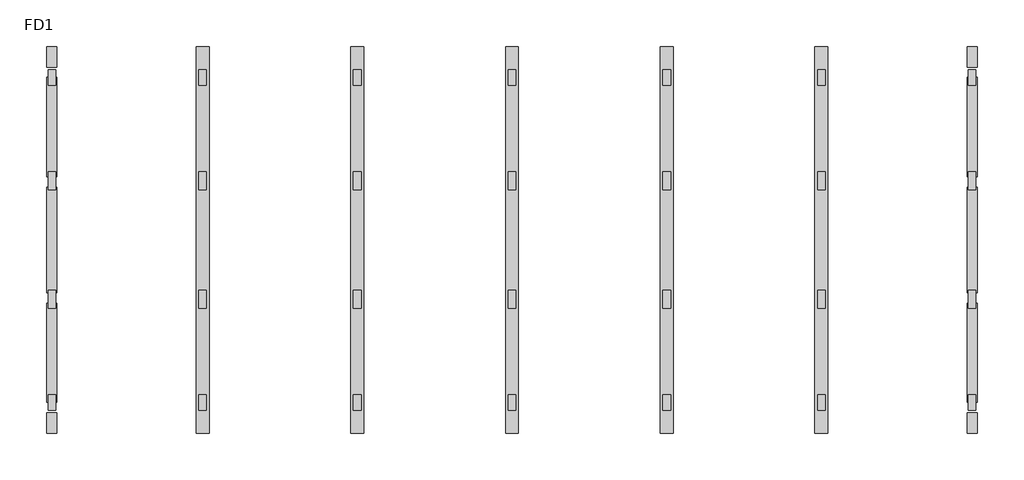
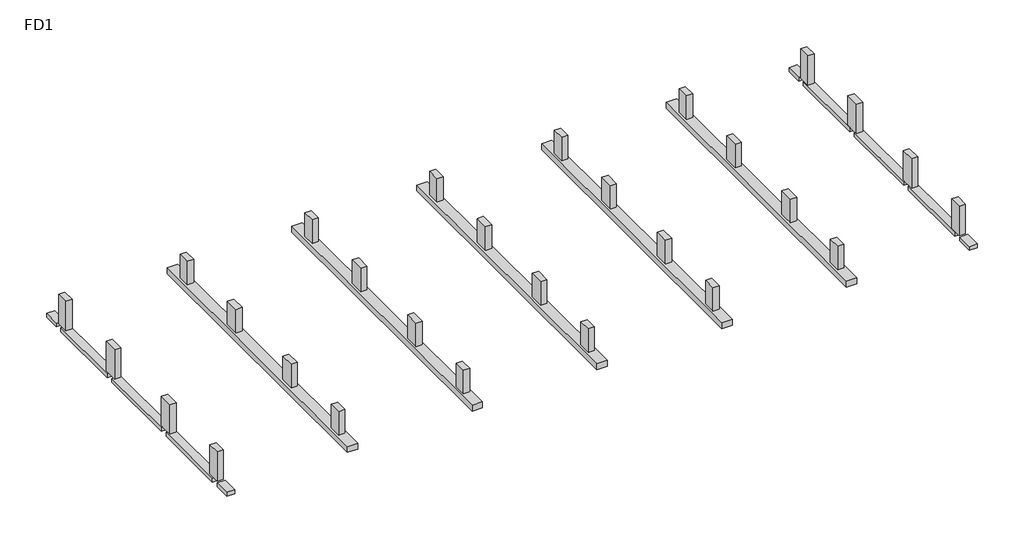
# One storey: 28 columns, 7 beams.
"""IFC4 building model written with IfcOpenShell, lengths in millimetres."""

from ifc_helpers import new_model, si_unit, frame, origin, place, context, project, spatial, polyline, outline, extrude, faceted_brep, element, save

model = new_model("IFC4")

# Units and contexts
model_context = context("Model", 3, world=origin())
ifc_project = project(units=[si_unit("LENGTHUNIT", "METRE", prefix="MILLI")], contexts=[model_context])

# Site, building, storey
site = spatial("IfcSite", under=ifc_project)
building = spatial("IfcBuilding", under=site)
storey = spatial("IfcBuildingStorey", under=building, Name="FD1", Elevation=-1170.0)

# Beams
placement = place(None, origin())
element("IfcBeam", 1, ObjectType="M_Concrete-Rectangular Beam : 400x700", at=placement, inside=storey, context=model_context, shape_type="SweptSolid", body=[
    extrude(outline(polyline([(35899.948043, -1000.0), (35499.948043, -1000.0), (35499.948043, -200.0), (35899.948043, -200.0), (35899.948043, -1000.0)])), frame((0.0, 0.0, -1670.0), z_axis=(0.0, 0.0, 1.0), x_axis=(1.0, 0.0, 0.0)), (0.0, 0.0, 1.0), 200.0),
    extrude(outline(polyline([(35499.948043, 14000.0000002), (35899.948043, 14000.0000002), (35899.948043, 13200.0000002), (35499.948043, 13200.0000002), (35499.948043, 14000.0000002)])), frame((0.0, 0.0, -1670.0), z_axis=(0.0, 0.0, 1.0), x_axis=(1.0, 0.0, 0.0)), (0.0, 0.0, 1.0), 200.0),
    extrude(outline(polyline([(35499.948043, 12800.0000002), (35899.948043, 12800.0000002), (35899.948043, 8950.0000002), (35499.948043, 8950.0000002), (35499.948043, 12800.0000002)])), frame((0.0, 0.0, -1670.0), z_axis=(0.0, 0.0, 1.0), x_axis=(1.0, 0.0, 0.0)), (0.0, 0.0, 1.0), 200.0),
    extrude(outline(polyline([(35499.948043, 8550.0000002), (35899.948043, 8550.0000002), (35899.948043, 4450.0000002), (35499.948043, 4450.0000002), (35499.948043, 8550.0000002)])), frame((0.0, 0.0, -1670.0), z_axis=(0.0, 0.0, 1.0), x_axis=(1.0, 0.0, 0.0)), (0.0, 0.0, 1.0), 200.0),
    extrude(outline(polyline([(35499.948043, 4050.0000002), (35899.948043, 4050.0000002), (35899.948043, 200.0), (35499.948043, 200.0), (35499.948043, 4050.0000002)])), frame((0.0, 0.0, -1670.0), z_axis=(0.0, 0.0, 1.0), x_axis=(1.0, 0.0, 0.0)), (0.0, 0.0, 1.0), 200.0),
])
element("IfcBeam", 2, ObjectType="M_Concrete-Rectangular Beam : 400x700", at=placement, inside=storey, context=model_context, shape_type="SweptSolid", body=[
    extrude(outline(polyline([(200.0, -1000.0), (-200.0, -1000.0), (-200.0, -200.0), (200.0, -200.0), (200.0, -1000.0)])), frame((0.0, 0.0, -1670.0), z_axis=(0.0, 0.0, 1.0), x_axis=(1.0, 0.0, 0.0)), (0.0, 0.0, 1.0), 200.0),
    extrude(outline(polyline([(-200.0, 14000.0000002), (200.0, 14000.0000002), (200.0, 13200.0000002), (-200.0, 13200.0000002), (-200.0, 14000.0000002)])), frame((0.0, 0.0, -1670.0), z_axis=(0.0, 0.0, 1.0), x_axis=(1.0, 0.0, 0.0)), (0.0, 0.0, 1.0), 200.0),
    extrude(outline(polyline([(-200.0, 12800.0000002), (200.0, 12800.0000002), (200.0, 8950.0000002), (-200.0, 8950.0000002), (-200.0, 12800.0000002)])), frame((0.0, 0.0, -1670.0), z_axis=(0.0, 0.0, 1.0), x_axis=(1.0, 0.0, 0.0)), (0.0, 0.0, 1.0), 200.0),
    extrude(outline(polyline([(-200.0, 8550.0000002), (200.0, 8550.0000002), (200.0, 4450.0000002), (-200.0, 4450.0000002), (-200.0, 8550.0000002)])), frame((0.0, 0.0, -1670.0), z_axis=(0.0, 0.0, 1.0), x_axis=(1.0, 0.0, 0.0)), (0.0, 0.0, 1.0), 200.0),
    extrude(outline(polyline([(-200.0, 4050.0000002), (200.0, 4050.0000002), (200.0, 200.0), (-200.0, 200.0), (-200.0, 4050.0000002)])), frame((0.0, 0.0, -1670.0), z_axis=(0.0, 0.0, 1.0), x_axis=(1.0, 0.0, 0.0)), (0.0, 0.0, 1.0), 200.0),
])
element("IfcBeam", 3, ObjectType="M_Concrete-Rectangular Beam : 500x1000", at=placement, inside=storey, context=model_context, shape_type="SweptSolid", body=[
    extrude(outline(polyline([(29600.0000039, 14000.0000002), (30100.0000039, 14000.0000002), (30100.0000039, -1000.0), (29600.0000039, -1000.0), (29600.0000039, 14000.0000002)])), frame((0.0, 0.0, -1470.0), z_axis=(0.0, 0.0, 1.0), x_axis=(1.0, 0.0, 0.0)), (0.0, 0.0, 1.0), 300.0),
])
element("IfcBeam", 4, ObjectType="M_Concrete-Rectangular Beam : 500x1000", at=placement, inside=storey, context=model_context, shape_type="SweptSolid", body=[
    extrude(outline(polyline([(6100.0000012, -1000.0), (5600.0000012, -1000.0), (5600.0000012, 14000.0000002), (6100.0000012, 14000.0000002), (6100.0000012, -1000.0)])), frame((0.0, 0.0, -1470.0), z_axis=(0.0, 0.0, 1.0), x_axis=(1.0, 0.0, 0.0)), (0.0, 0.0, 1.0), 300.0),
])
element("IfcBeam", 5, ObjectType="M_Concrete-Rectangular Beam : 500x1000", at=placement, inside=storey, context=model_context, shape_type="Brep", body=[
    faceted_brep([(24100.0000056, -1000.0, -1170.0), (23600.0000056, -1000.0, -1170.0), (23600.0000056, -1000.0, -1469.9652093), (24100.0000056, -1000.0, -1470.0), (23600.0000056, 14000.0000002, -1170.0), (24100.0000056, 14000.0000002, -1170.0), (24100.0000056, 14000.0000002, -1470.0347907), (23600.0000056, 14000.0000002, -1470.0)], [[[0, 1, 2, 3]], [[4, 5, 6, 7]], [[1, 0, 5, 4]], [[1, 4, 7, 2]], [[5, 0, 3, 6]], [[3, 2, 7, 6]]]),
])
element("IfcBeam", 6, ObjectType="M_Concrete-Rectangular Beam : 500x1000", at=placement, inside=storey, context=model_context, shape_type="Brep", body=[
    faceted_brep([(18099.8537458, -1000.0, -1170.0), (17599.8537458, -1000.0, -1170.0), (17599.8537458, -1000.0, -1469.962184), (18099.8537458, -1000.0, -1470.0), (17599.8537458, 14000.0000002, -1170.0), (18099.8537458, 14000.0000002, -1170.0), (18099.8537458, 14000.0000002, -1470.037816), (17599.8537458, 14000.0000002, -1470.0)], [[[0, 1, 2, 3]], [[4, 5, 6, 7]], [[1, 0, 5, 4]], [[1, 4, 7, 2]], [[5, 0, 3, 6]], [[3, 2, 7, 6]]]),
])
element("IfcBeam", 7, ObjectType="M_Concrete-Rectangular Beam : 500x1000", at=placement, inside=storey, context=model_context, shape_type="Brep", body=[
    faceted_brep([(12100.0000006, -1000.0, -1170.0), (11600.0000006, -1000.0, -1170.0), (11600.0000006, -1000.0, -1469.9652093), (12100.0000006, -1000.0, -1470.0), (11600.0000006, 14000.0000002, -1170.0), (12100.0000006, 14000.0000002, -1170.0), (12100.0000006, 14000.0000002, -1470.0347907), (11600.0000006, 14000.0000002, -1470.0)], [[[0, 1, 2, 3]], [[4, 5, 6, 7]], [[1, 0, 5, 4]], [[1, 4, 7, 2]], [[5, 0, 3, 6]], [[3, 2, 7, 6]]]),
])

# Columns
element("IfcColumn", 8, ObjectType="M_Concrete-Rectangular-Column : 300x600", at=placement, inside=storey, context=model_context, shape_type="SweptSolid", body=[
    extrude(outline(polyline([(165.0, 499.9999998), (165.0, -100.0000002), (-135.0, -100.0000002), (-135.0, 499.9999998), (165.0, 499.9999998)])), frame((0.0, 0.0, -1470.0), z_axis=(0.0, 0.0, 1.0), x_axis=(1.0, 0.0, 0.0)), (0.0, 0.0, 1.0), 1500.0),
])
element("IfcColumn", 9, ObjectType="M_Concrete-Rectangular-Column : 300x600", at=placement, inside=storey, context=model_context, shape_type="SweptSolid", body=[
    extrude(outline(polyline([(164.9999993, 13100.0000003), (164.9999993, 12500.0000003), (-135.0000007, 12500.0000003), (-135.0000007, 13100.0000003), (164.9999993, 13100.0000003)])), frame((0.0, 0.0, -1470.0), z_axis=(0.0, 0.0, 1.0), x_axis=(1.0, 0.0, 0.0)), (0.0, 0.0, 1.0), 1500.0),
])
element("IfcColumn", 10, ObjectType="M_Concrete-Rectangular-Column : 300x600", at=placement, inside=storey, context=model_context, shape_type="SweptSolid", body=[
    extrude(outline(polyline([(6000.0000007, 499.9999998), (6000.0000007, -100.0000002), (5700.0000007, -100.0000002), (5700.0000007, 499.9999998), (6000.0000007, 499.9999998)])), frame((0.0, 0.0, -1170.0), z_axis=(0.0, 0.0, 1.0), x_axis=(1.0, 0.0, 0.0)), (0.0, 0.0, 1.0), 1200.0),
])
element("IfcColumn", 11, ObjectType="M_Concrete-Rectangular-Column : 300x600", at=placement, inside=storey, context=model_context, shape_type="SweptSolid", body=[
    extrude(outline(polyline([(12000.0000034, 499.9999998), (12000.0000034, -100.0000002), (11700.0000034, -100.0000002), (11700.0000034, 499.9999998), (12000.0000034, 499.9999998)])), frame((0.0, 0.0, -1170.0), z_axis=(0.0, 0.0, 1.0), x_axis=(1.0, 0.0, 0.0)), (0.0, 0.0, 1.0), 1200.0),
])
element("IfcColumn", 12, ObjectType="M_Concrete-Rectangular-Column : 300x600", at=placement, inside=storey, context=model_context, shape_type="SweptSolid", body=[
    extrude(outline(polyline([(18000.0000058, 499.9999998), (18000.0000058, -100.0000002), (17700.0000058, -100.0000002), (17700.0000058, 499.9999998), (18000.0000058, 499.9999998)])), frame((0.0, 0.0, -1170.0), z_axis=(0.0, 0.0, 1.0), x_axis=(1.0, 0.0, 0.0)), (0.0, 0.0, 1.0), 1200.0),
])
element("IfcColumn", 13, ObjectType="M_Concrete-Rectangular-Column : 300x600", at=placement, inside=storey, context=model_context, shape_type="SweptSolid", body=[
    extrude(outline(polyline([(24000.0000047, 499.9999998), (24000.0000047, -100.0000002), (23700.0000047, -100.0000002), (23700.0000047, 499.9999998), (24000.0000047, 499.9999998)])), frame((0.0, 0.0, -1170.0), z_axis=(0.0, 0.0, 1.0), x_axis=(1.0, 0.0, 0.0)), (0.0, 0.0, 1.0), 1200.0),
])
element("IfcColumn", 14, ObjectType="M_Concrete-Rectangular-Column : 300x600", at=placement, inside=storey, context=model_context, shape_type="SweptSolid", body=[
    extrude(outline(polyline([(6000.0000007, 13100.0000003), (6000.0000007, 12500.0000003), (5700.0000007, 12500.0000003), (5700.0000007, 13100.0000003), (6000.0000007, 13100.0000003)])), frame((0.0, 0.0, -1170.0), z_axis=(0.0, 0.0, 1.0), x_axis=(1.0, 0.0, 0.0)), (0.0, 0.0, 1.0), 1200.0),
])
element("IfcColumn", 15, ObjectType="M_Concrete-Rectangular-Column : 300x600", at=placement, inside=storey, context=model_context, shape_type="SweptSolid", body=[
    extrude(outline(polyline([(12000.0000034, 13100.0000003), (12000.0000034, 12500.0000003), (11700.0000034, 12500.0000003), (11700.0000034, 13100.0000003), (12000.0000034, 13100.0000003)])), frame((0.0, 0.0, -1170.0), z_axis=(0.0, 0.0, 1.0), x_axis=(1.0, 0.0, 0.0)), (0.0, 0.0, 1.0), 1200.0),
])
element("IfcColumn", 16, ObjectType="M_Concrete-Rectangular-Column : 300x600", at=placement, inside=storey, context=model_context, shape_type="SweptSolid", body=[
    extrude(outline(polyline([(18000.0000058, 13100.0000003), (18000.0000058, 12500.0000003), (17700.0000058, 12500.0000003), (17700.0000058, 13100.0000003), (18000.0000058, 13100.0000003)])), frame((0.0, 0.0, -1170.0), z_axis=(0.0, 0.0, 1.0), x_axis=(1.0, 0.0, 0.0)), (0.0, 0.0, 1.0), 1200.0),
])
element("IfcColumn", 17, ObjectType="M_Concrete-Rectangular-Column : 300x600", at=placement, inside=storey, context=model_context, shape_type="SweptSolid", body=[
    extrude(outline(polyline([(24000.0000047, 13100.0000003), (24000.0000047, 12500.0000003), (23700.0000047, 12500.0000003), (23700.0000047, 13100.0000003), (24000.0000047, 13100.0000003)])), frame((0.0, 0.0, -1170.0), z_axis=(0.0, 0.0, 1.0), x_axis=(1.0, 0.0, 0.0)), (0.0, 0.0, 1.0), 1200.0),
])
element("IfcColumn", 18, ObjectType="M_Concrete-Rectangular-Column : 300x600", at=placement, inside=storey, context=model_context, shape_type="SweptSolid", body=[
    extrude(outline(polyline([(30000.0000039, 499.9999998), (30000.0000039, -100.0000002), (29700.0000039, -100.0000002), (29700.0000039, 499.9999998), (30000.0000039, 499.9999998)])), frame((0.0, 0.0, -1170.0), z_axis=(0.0, 0.0, 1.0), x_axis=(1.0, 0.0, 0.0)), (0.0, 0.0, 1.0), 1200.0),
])
element("IfcColumn", 19, ObjectType="M_Concrete-Rectangular-Column : 300x600", at=placement, inside=storey, context=model_context, shape_type="SweptSolid", body=[
    extrude(outline(polyline([(30000.0000039, 13100.0000003), (30000.0000039, 12500.0000003), (29700.0000039, 12500.0000003), (29700.0000039, 13100.0000003), (30000.0000039, 13100.0000003)])), frame((0.0, 0.0, -1170.0), z_axis=(0.0, 0.0, 1.0), x_axis=(1.0, 0.0, 0.0)), (0.0, 0.0, 1.0), 1200.0),
])
element("IfcColumn", 20, ObjectType="M_Concrete-Rectangular-Column : 300x600", at=placement, inside=storey, context=model_context, shape_type="SweptSolid", body=[
    extrude(outline(polyline([(35835.035019, 499.9999998), (35835.035019, -100.0000002), (35535.035019, -100.0000002), (35535.035019, 499.9999998), (35835.035019, 499.9999998)])), frame((0.0, 0.0, -1470.0), z_axis=(0.0, 0.0, 1.0), x_axis=(1.0, 0.0, 0.0)), (0.0, 0.0, 1.0), 1500.0),
])
element("IfcColumn", 21, ObjectType="M_Concrete-Rectangular-Column : 300x600", at=placement, inside=storey, context=model_context, shape_type="SweptSolid", body=[
    extrude(outline(polyline([(35835.035019, 13100.0000003), (35835.035019, 12500.0000003), (35535.035019, 12500.0000003), (35535.035019, 13100.0000003), (35835.035019, 13100.0000003)])), frame((0.0, 0.0, -1470.0), z_axis=(0.0, 0.0, 1.0), x_axis=(1.0, 0.0, 0.0)), (0.0, 0.0, 1.0), 1500.0),
])
element("IfcColumn", 22, ObjectType="M_Concrete-Rectangular-Column : 300x700", at=placement, inside=storey, context=model_context, shape_type="SweptSolid", body=[
    extrude(outline(polyline([(165.0, 4550.0000002), (165.0, 3850.0000002), (-135.0, 3850.0000002), (-135.0, 4550.0000002), (165.0, 4550.0000002)])), frame((0.0, 0.0, -1470.0), z_axis=(0.0, 0.0, 1.0), x_axis=(1.0, 0.0, 0.0)), (0.0, 0.0, 1.0), 1500.0),
])
element("IfcColumn", 23, ObjectType="M_Concrete-Rectangular-Column : 300x700", at=placement, inside=storey, context=model_context, shape_type="SweptSolid", body=[
    extrude(outline(polyline([(165.0, 9149.9985388), (165.0, 8449.9985388), (-135.0, 8449.9985388), (-135.0, 9149.9985388), (165.0, 9149.9985388)])), frame((0.0, 0.0, -1470.0), z_axis=(0.0, 0.0, 1.0), x_axis=(1.0, 0.0, 0.0)), (0.0, 0.0, 1.0), 1500.0),
])
element("IfcColumn", 24, ObjectType="M_Concrete-Rectangular-Column : 300x700", at=placement, inside=storey, context=model_context, shape_type="SweptSolid", body=[
    extrude(outline(polyline([(6000.0000007, 4550.0000002), (6000.0000007, 3850.0000002), (5700.0000007, 3850.0000002), (5700.0000007, 4550.0000002), (6000.0000007, 4550.0000002)])), frame((0.0, 0.0, -1170.0), z_axis=(0.0, 0.0, 1.0), x_axis=(1.0, 0.0, 0.0)), (0.0, 0.0, 1.0), 1200.0),
])
element("IfcColumn", 25, ObjectType="M_Concrete-Rectangular-Column : 300x700", at=placement, inside=storey, context=model_context, shape_type="SweptSolid", body=[
    extrude(outline(polyline([(12000.0000034, 4550.0000002), (12000.0000034, 3850.0000002), (11700.0000034, 3850.0000002), (11700.0000034, 4550.0000002), (12000.0000034, 4550.0000002)])), frame((0.0, 0.0, -1170.0), z_axis=(0.0, 0.0, 1.0), x_axis=(1.0, 0.0, 0.0)), (0.0, 0.0, 1.0), 1200.0),
])
element("IfcColumn", 26, ObjectType="M_Concrete-Rectangular-Column : 300x700", at=placement, inside=storey, context=model_context, shape_type="SweptSolid", body=[
    extrude(outline(polyline([(18000.0000058, 4550.0000002), (18000.0000058, 3850.0000002), (17700.0000058, 3850.0000002), (17700.0000058, 4550.0000002), (18000.0000058, 4550.0000002)])), frame((0.0, 0.0, -1170.0), z_axis=(0.0, 0.0, 1.0), x_axis=(1.0, 0.0, 0.0)), (0.0, 0.0, 1.0), 1200.0),
])
element("IfcColumn", 27, ObjectType="M_Concrete-Rectangular-Column : 300x700", at=placement, inside=storey, context=model_context, shape_type="SweptSolid", body=[
    extrude(outline(polyline([(24000.0000047, 4550.0000002), (24000.0000047, 3850.0000002), (23700.0000047, 3850.0000002), (23700.0000047, 4550.0000002), (24000.0000047, 4550.0000002)])), frame((0.0, 0.0, -1170.0), z_axis=(0.0, 0.0, 1.0), x_axis=(1.0, 0.0, 0.0)), (0.0, 0.0, 1.0), 1200.0),
])
element("IfcColumn", 28, ObjectType="M_Concrete-Rectangular-Column : 300x700", at=placement, inside=storey, context=model_context, shape_type="SweptSolid", body=[
    extrude(outline(polyline([(6000.0000007, 9149.9985388), (6000.0000007, 8449.9985388), (5700.0000007, 8449.9985388), (5700.0000007, 9149.9985388), (6000.0000007, 9149.9985388)])), frame((0.0, 0.0, -1170.0), z_axis=(0.0, 0.0, 1.0), x_axis=(1.0, 0.0, 0.0)), (0.0, 0.0, 1.0), 1200.0),
])
element("IfcColumn", 29, ObjectType="M_Concrete-Rectangular-Column : 300x700", at=placement, inside=storey, context=model_context, shape_type="SweptSolid", body=[
    extrude(outline(polyline([(12000.0000034, 9149.9985388), (12000.0000034, 8449.9985388), (11700.0000034, 8449.9985388), (11700.0000034, 9149.9985388), (12000.0000034, 9149.9985388)])), frame((0.0, 0.0, -1170.0), z_axis=(0.0, 0.0, 1.0), x_axis=(1.0, 0.0, 0.0)), (0.0, 0.0, 1.0), 1200.0),
])
element("IfcColumn", 30, ObjectType="M_Concrete-Rectangular-Column : 300x700", at=placement, inside=storey, context=model_context, shape_type="SweptSolid", body=[
    extrude(outline(polyline([(18000.0000058, 9149.9985388), (18000.0000058, 8449.9985388), (17700.0000058, 8449.9985388), (17700.0000058, 9149.9985388), (18000.0000058, 9149.9985388)])), frame((0.0, 0.0, -1170.0), z_axis=(0.0, 0.0, 1.0), x_axis=(1.0, 0.0, 0.0)), (0.0, 0.0, 1.0), 1200.0),
])
element("IfcColumn", 31, ObjectType="M_Concrete-Rectangular-Column : 300x700", at=placement, inside=storey, context=model_context, shape_type="SweptSolid", body=[
    extrude(outline(polyline([(24000.0000047, 9149.9985388), (24000.0000047, 8449.9985388), (23700.0000047, 8449.9985388), (23700.0000047, 9149.9985388), (24000.0000047, 9149.9985388)])), frame((0.0, 0.0, -1170.0), z_axis=(0.0, 0.0, 1.0), x_axis=(1.0, 0.0, 0.0)), (0.0, 0.0, 1.0), 1200.0),
])
element("IfcColumn", 32, ObjectType="M_Concrete-Rectangular-Column : 300x700", at=placement, inside=storey, context=model_context, shape_type="SweptSolid", body=[
    extrude(outline(polyline([(30000.0000039, 4550.0000002), (30000.0000039, 3850.0000002), (29700.0000039, 3850.0000002), (29700.0000039, 4550.0000002), (30000.0000039, 4550.0000002)])), frame((0.0, 0.0, -1170.0), z_axis=(0.0, 0.0, 1.0), x_axis=(1.0, 0.0, 0.0)), (0.0, 0.0, 1.0), 1200.0),
])
element("IfcColumn", 33, ObjectType="M_Concrete-Rectangular-Column : 300x700", at=placement, inside=storey, context=model_context, shape_type="SweptSolid", body=[
    extrude(outline(polyline([(30000.0000039, 9149.9985388), (30000.0000039, 8449.9985388), (29700.0000039, 8449.9985388), (29700.0000039, 9149.9985388), (30000.0000039, 9149.9985388)])), frame((0.0, 0.0, -1170.0), z_axis=(0.0, 0.0, 1.0), x_axis=(1.0, 0.0, 0.0)), (0.0, 0.0, 1.0), 1200.0),
])
element("IfcColumn", 34, ObjectType="M_Concrete-Rectangular-Column : 300x700", at=placement, inside=storey, context=model_context, shape_type="SweptSolid", body=[
    extrude(outline(polyline([(35834.7667691, 4550.0000002), (35834.7667691, 3850.0000002), (35534.7667691, 3850.0000002), (35534.7667691, 4550.0000002), (35834.7667691, 4550.0000002)])), frame((0.0, 0.0, -1470.0), z_axis=(0.0, 0.0, 1.0), x_axis=(1.0, 0.0, 0.0)), (0.0, 0.0, 1.0), 1500.0),
])
element("IfcColumn", 35, ObjectType="M_Concrete-Rectangular-Column : 300x700", at=placement, inside=storey, context=model_context, shape_type="SweptSolid", body=[
    extrude(outline(polyline([(35835.035019, 9149.9985388), (35835.035019, 8449.9985388), (35535.035019, 8449.9985388), (35535.035019, 9149.9985388), (35835.035019, 9149.9985388)])), frame((0.0, 0.0, -1470.0), z_axis=(0.0, 0.0, 1.0), x_axis=(1.0, 0.0, 0.0)), (0.0, 0.0, 1.0), 1500.0),
])

save(model, "model.ifc")

# Revit data of these elements
# Type "M_Concrete-Rectangular Beam : 400x700"
#   Length [instance default] = 1524 mm
#   b = 400 mm
#   h = 700 mm
#   Structural Material [instance default] = Concrete, Cast-in-Place gray
#   Assembly Code = ""
# Type "M_Concrete-Rectangular Beam : 500x1000"
#   Length [instance default] = 1524 mm
#   b = 500 mm
#   h = 1000 mm
#   Structural Material [instance default] = Concrete, Cast-in-Place gray
#   Assembly Code = ""
# Type "M_Concrete-Rectangular-Column : 300x600"
#   b = 300 mm
#   h = 600 mm
#   Structural Material [instance default] = Concrete, Cast-in-Place gray
# Type "M_Concrete-Rectangular-Column : 300x700"
#   b = 300 mm
#   h = 700 mm
#   Structural Material [instance default] = Concrete, Cast-in-Place gray
# Elements 1, 2 (IfcBeam, "M_Concrete-Rectangular Beam : 400x700")
#   Comments = ""
#   Structural Material = Concrete, Cast-in-Place gray
#   Phase Created = New Construction
#   Materials on its faces: "Concrete, Cast-in-Place gray"
# Elements 3, 4, 5, 6, 7 (IfcBeam, "M_Concrete-Rectangular Beam : 500x1000")
#   Comments = ""
#   Structural Material = Concrete, Cast-in-Place gray
#   Phase Created = New Construction
#   Materials on its faces: "Concrete, Cast-in-Place gray"
# Elements 8, 9, 10, 11, 13, 14, 15, 17, 18, 19, 20, 21 (IfcColumn, "M_Concrete-Rectangular-Column : 300x600")
#   Comments = ""
#   COF_CON__WorkItemNumber = "SH3-A-GF"
#   COF_GEN__Name = "CC1"
#   Structural Material = Concrete, Cast-in-Place gray
#   Phase Created = New Construction
#   Materials on its faces: "Concrete, Cast-in-Place gray"
# Elements 12, 16 (IfcColumn, "M_Concrete-Rectangular-Column : 300x600")
#   Comments = ""
#   COF_CON__WorkItemNumber = "SH3-A-GF"
#   COF_GEN__Name = "CC2"
#   Structural Material = Concrete, Cast-in-Place gray
#   Phase Created = New Construction
#   Materials on its faces: "Concrete, Cast-in-Place gray"
# Elements 22, 23, 34, 35 (IfcColumn, "M_Concrete-Rectangular-Column : 300x700")
#   Comments = ""
#   COF_CON__WorkItemNumber = "SH3-A-GF"
#   COF_GEN__Name = "CC3"
#   Structural Material = Concrete, Cast-in-Place gray
#   Phase Created = New Construction
#   Materials on its faces: "Concrete, Cast-in-Place gray"
# Elements 24, 28, 32, 33 (IfcColumn, "M_Concrete-Rectangular-Column : 300x700")
#   Comments = ""
#   COF_CON__WorkItemNumber = "SH3-A-GF"
#   COF_GEN__Name = "CC4"
#   Structural Material = Concrete, Cast-in-Place gray
#   Phase Created = New Construction
#   Materials on its faces: "Concrete, Cast-in-Place gray"
# Elements 25, 27, 29, 31 (IfcColumn, "M_Concrete-Rectangular-Column : 300x700")
#   Comments = ""
#   COF_CON__WorkItemNumber = "SH3-A-GF"
#   COF_GEN__Name = "CC5"
#   Structural Material = Concrete, Cast-in-Place gray
#   Phase Created = New Construction
#   Materials on its faces: "Concrete, Cast-in-Place gray"
# Elements 26, 30 (IfcColumn, "M_Concrete-Rectangular-Column : 300x700")
#   Comments = ""
#   COF_CON__WorkItemNumber = "SH3-A-GF"
#   COF_GEN__Name = "CC6"
#   Structural Material = Concrete, Cast-in-Place gray
#   Phase Created = New Construction
#   Materials on its faces: "Concrete, Cast-in-Place gray"
# Materials
#   "Concrete, Cast-in-Place gray": class "Concrete", colour RGB 207 208 204, transparency 0, Description = "Cast-in-place concrete", Cost = 0
